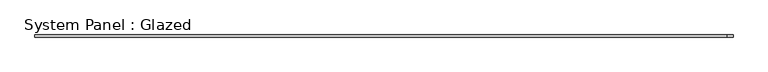
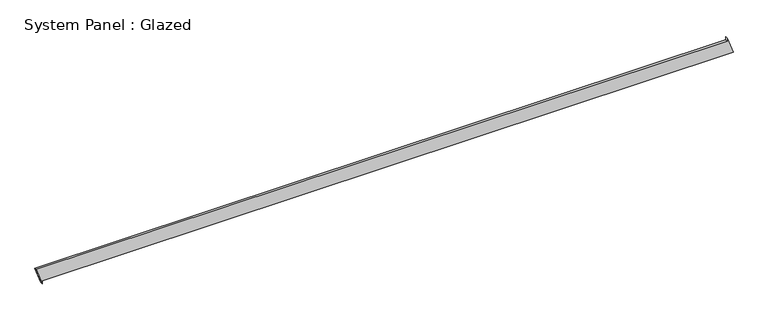
"""IFC4 building model written with IfcOpenShell, lengths in millimetres: plate geometry, System Panel : Glazed."""

from ifc_helpers import new_model, si_unit, frame, origin, place, context, project, spatial, polyline, outline, extrude, source, transform, mapped, element, save


def system_panel_glazed_2a14b6e4(model_context):
    return source(origin(), model_context, "Body", "SweptSolid", [
        extrude(outline(polyline([(0.0, -3958.4240501), (35.3553391, -3958.4240501), (35.3553391, 4028.218169), (234.3325301, 3958.5389074), (198.9771911, 3958.5391215), (198.928805, -4028.218169), (0.0, -3958.4240501)])), frame((0.0, -49.5, 0.0), z_axis=(0.0, 1.0, 0.0), x_axis=(0.0, 0.0, 1.0)), (0.0, 0.0, 1.0), 25.0),
    ])


if __name__ == "__main__":
    model = new_model("IFC4")
    model_context = context("Model", 3, world=origin())
    ifc_project = project(units=[si_unit("LENGTHUNIT", "METRE", prefix="MILLI")], contexts=[model_context])
    site = spatial("IfcSite", under=ifc_project)
    building = spatial("IfcBuilding", under=site)
    placement = place(None, origin())
    system_panel_glazed_shape = system_panel_glazed_2a14b6e4(model_context)
    element("IfcPlate", 1, ObjectType="System Panel : Glazed", at=placement, inside=building, context=model_context, shape_type="MappedRepresentation", body=[
        mapped(system_panel_glazed_shape, transform((0.0, 0.0, 0.0), x_axis=(1.0, 0.0, 0.0), y_axis=(0.0, 1.0, 0.0), z_axis=(0.0, 0.0, 1.0))),
    ])
    save(model, "model.ifc")

# Revit data of these elements
# Element 1 (IfcPlate, "System Panel : Glazed")
#   Materials on its faces: "Glass"
# Materials
#   "Glass": class "Glass", colour RGB 218 227 224, transparency 0.85, Description = "Soda Lime Glass", Cost = 0
